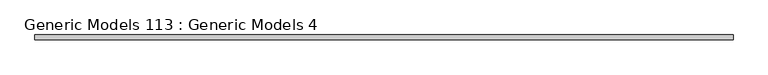
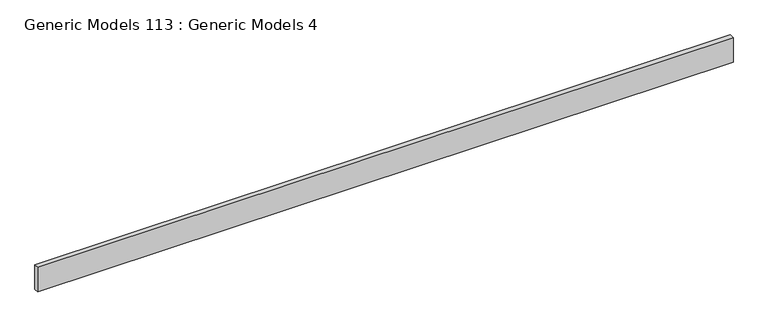
"""IFC4 building model written with IfcOpenShell, lengths in millimetres: proxy geometry, Generic Models 113 : Generic Models 4."""

from ifc_helpers import new_model, si_unit, frame, origin, place, context, project, spatial, polyline, outline, extrude, source, transform, mapped, element, save


def generic_models_113_generic_models_4_ef66705d(model_context):
    return source(origin(), model_context, "Body", "SweptSolid", [
        extrude(outline(polyline([(8544.7579126, 7029.4078185), (8544.7579126, 6902.4078185), (-10098.8420874, 6902.4078185), (-10098.8420874, 7029.4078185), (8544.7579126, 7029.4078185)])), frame((0.0, 0.0, 123466.5552725), z_axis=(0.0, 0.0, 1.0), x_axis=(1.0, 0.0, 0.0)), (0.0, 0.0, 1.0), 694.4038478),
    ])


if __name__ == "__main__":
    model = new_model("IFC4")
    model_context = context("Model", 3, world=origin())
    ifc_project = project(units=[si_unit("LENGTHUNIT", "METRE", prefix="MILLI")], contexts=[model_context])
    site = spatial("IfcSite", under=ifc_project)
    building = spatial("IfcBuilding", under=site)
    placement = place(None, origin())
    generic_models_113_generic_models_4_shape = generic_models_113_generic_models_4_ef66705d(model_context)
    element("IfcBuildingElementProxy", 1, Name="Generic Models 113 : Generic Models 4", ObjectType="Generic Models 113 : Generic Models 4", at=placement, inside=building, context=model_context, shape_type="MappedRepresentation", body=[
        mapped(generic_models_113_generic_models_4_shape, transform((0.0, 0.0, 0.0), x_axis=(1.0, 0.0, 0.0), y_axis=(0.0, 1.0, 0.0), z_axis=(0.0, 0.0, 1.0))),
    ])
    save(model, "model.ifc")

# Revit data of these elements
# Element 1 (IfcBuildingElementProxy, "Generic Models 113 : Generic Models 4")
#   Materials on its faces: "_BATT INSUL. (U-FACTOR = 0.065 MIN.) OVER CLASS II VAPOR RETARDER(TOWARD INTERIOR)"
# Materials
#   "_BATT INSUL. (U-FACTOR = 0.065 MIN.) OVER CLASS II VAPOR RETARDER(TOWARD INTERIOR)": class "Generic", colour RGB 227 210 251, transparency 0, Cost = 0
